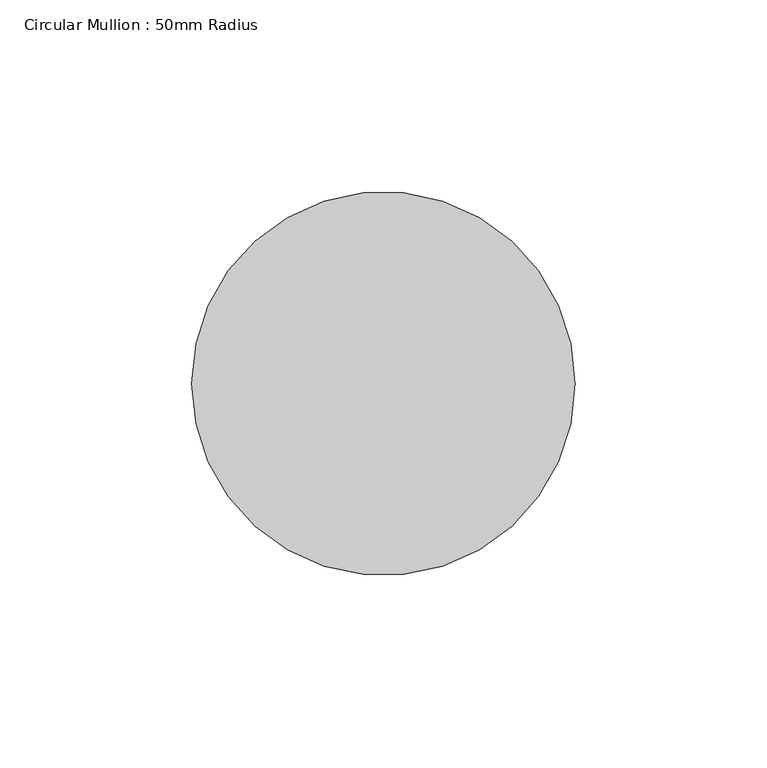
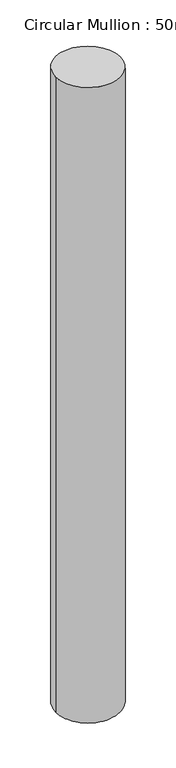
"""IFC4 building model written with IfcOpenShell, lengths in millimetres: member geometry, Circular Mullion : 50mm Radius."""

from ifc_helpers import new_model, si_unit, frame, origin, place, context, project, spatial, ellipse_curve, source, transform, mapped, element, save
from ifc_brep_helpers import plane_surface, cylinder_surface, advanced_brep


def circular_mullion_50mm_radius_0e1b4e99(model_context):
    return source(origin(), model_context, "Body", "AdvancedBrep", [
        advanced_brep(
        [(-100.0, 0.0, 1.4218944), (0.0, 0.0, 0.0), (0.0, 0.0, -1040.2054441), (-100.0, 0.0, -1041.6586869)],
        [
            (0, 1, ellipse_curve(frame((-50.0, 0.0, 0.7109472), z_axis=(-0.014215865107340957, -0.015196295125305462, -0.9997834674536855), x_axis=(-0.6830085911358856, -0.7301138584003781, 0.020809089511203346)), 50.010829, 50.0)),
            (1, 2),
            (2, 3, ellipse_curve(frame((-50.0, 0.0, -1040.9320655), z_axis=(-0.014529141967538954, -0.01553117784876709, 0.9997738176949411), x_axis=(0.6830019988402951, 0.7301068114519129, 0.021267662111344076)), 50.0113117, 50.0)),
            (3, 0),
            (1, 0, ellipse_curve(frame((-50.0, 0.0, 0.7109472), z_axis=(-0.014215865107340957, -0.015196295125305462, -0.9997834674536855), x_axis=(-0.6830085911358856, -0.7301138584003781, 0.020809089511203346)), 50.010829, 50.0)),
            (3, 2, ellipse_curve(frame((-50.0, 0.0, -1040.9320655), z_axis=(-0.014529141967538954, -0.01553117784876709, 0.9997738176949411), x_axis=(0.6830019988402951, 0.7301068114519129, 0.021267662111344076)), 50.0113117, 50.0)),
        ],
        [
            cylinder_surface(frame((-50.0, 0.0, 0.0), z_axis=(0.0, 0.0, 1.0), x_axis=(1.0, 0.0, 0.0)), 50.0),
            plane_surface(frame((-222.5869013, 208.2261063, 0.0), z_axis=(0.01421586510734096, 0.015196295125305466, 0.9997834674536857), x_axis=(0.6830085911358857, 0.730113858400378, -0.02080908951120872))),
            plane_surface(frame((-222.5869013, 208.2261063, -1040.2054441), z_axis=(0.01452914196753895, 0.015531177848767086, -0.9997738176949409), x_axis=(0.683001998840295, 0.7301068114519126, 0.021267662111358998))),
        ],
        [
            (0, [[1, 2, 3, 4]]),
            (0, [[5, -4, 6, -2]]),
            (1, [[-1, -5]]),
            (2, [[-6, -3]]),
        ],
    ),
    ])


if __name__ == "__main__":
    model = new_model("IFC4")
    model_context = context("Model", 3, world=origin())
    ifc_project = project(units=[si_unit("LENGTHUNIT", "METRE", prefix="MILLI")], contexts=[model_context])
    site = spatial("IfcSite", under=ifc_project)
    building = spatial("IfcBuilding", under=site)
    placement = place(None, origin())
    circular_mullion_50mm_radius_shape = circular_mullion_50mm_radius_0e1b4e99(model_context)
    element("IfcMember", 1, ObjectType="Circular Mullion : 50mm Radius", at=placement, inside=building, context=model_context, shape_type="MappedRepresentation", body=[
        mapped(circular_mullion_50mm_radius_shape, transform((0.0, 0.0, 0.0), x_axis=(1.0, 0.0, 0.0), y_axis=(0.0, 1.0, 0.0), z_axis=(0.0, 0.0, 1.0))),
    ])
    save(model, "model.ifc")

# Revit data of these elements
# Type "Circular Mullion : 50mm Radius"
#   built-in parameter 1007350 = 0.164042 (stored number, unit not read)
# Element 1 (IfcMember, "Circular Mullion : 50mm Radius")
#   Materials on its faces: "Aluminium"
# Materials
#   "Aluminium": class "Metal", colour RGB 247 247 247, transparency 0, Description = "Aluminium 6061", Cost = 0
